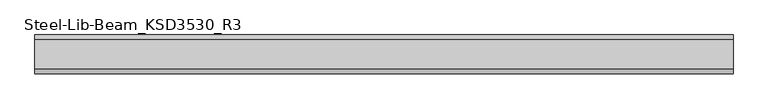
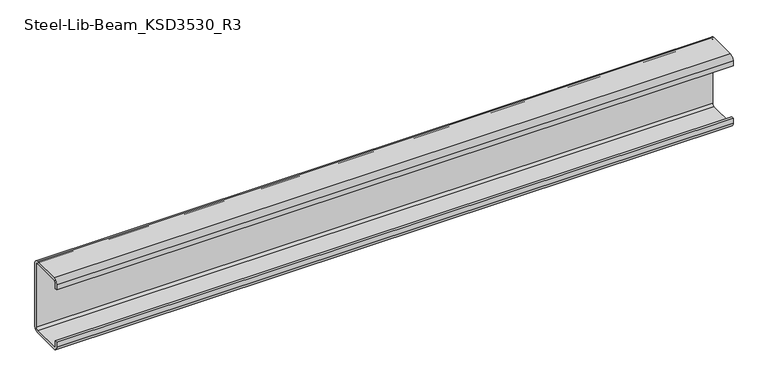
"""IFC4 building model written with IfcOpenShell, lengths in millimetres: beam geometry, Steel-Lib-Beam_KSD3530_R3 : BMS291_C-150×75x20x4.5."""

from ifc_helpers import new_model, si_unit, point, frame, frame_2d, origin, place, context, project, spatial, polyline, circle_curve, trimmed, segment, composite_curve, outline, extrude, source, transform, mapped, element, save


def steel_lib_beam_ksd3530_r3_1220318e(model_context):
    return source(origin(), model_context, "Body", "SweptSolid", [
        extrude(outline(composite_curve([segment(trimmed(circle_curve(frame_2d((-41.0, 66.0)), 9.0), [point((-50.0, 66.0))], [point((-41.0, 75.0))], False, "CARTESIAN"), True, "CONTINUOUS"), segment(polyline([(-41.0, 75.0), (16.0, 75.0)]), True, "CONTINUOUS"), segment(trimmed(circle_curve(frame_2d((16.0, 66.0)), 9.0), [point((16.0, 75.0))], [point((25.0, 66.0))], False, "CARTESIAN"), True, "CONTINUOUS"), segment(polyline([(25.0, 66.0), (25.0, -66.0)]), True, "CONTINUOUS"), segment(trimmed(circle_curve(frame_2d((16.0, -66.0)), 9.0), [point((25.0, -66.0))], [point((16.0, -75.0))], False, "CARTESIAN"), True, "CONTINUOUS"), segment(polyline([(16.0, -75.0), (-41.0, -75.0)]), True, "CONTINUOUS"), segment(trimmed(circle_curve(frame_2d((-41.0, -66.0)), 9.0), [point((-41.0, -75.0))], [point((-50.0, -66.0))], False, "CARTESIAN"), True, "CONTINUOUS"), segment(polyline([(-50.0, -66.0), (-50.0, -55.0), (-45.5, -55.0), (-45.5, -66.0)]), True, "CONTINUOUS"), segment(trimmed(circle_curve(frame_2d((-41.0, -66.0)), 4.5), [point((-45.5, -66.0))], [point((-41.0, -70.5))], True, "CARTESIAN"), True, "CONTINUOUS"), segment(polyline([(-41.0, -70.5), (16.0, -70.5)]), True, "CONTINUOUS"), segment(trimmed(circle_curve(frame_2d((16.0, -66.0)), 4.5), [point((16.0, -70.5))], [point((20.5, -66.0))], True, "CARTESIAN"), True, "CONTINUOUS"), segment(polyline([(20.5, -66.0), (20.5, 66.0)]), True, "CONTINUOUS"), segment(trimmed(circle_curve(frame_2d((16.0, 66.0)), 4.5), [point((20.5, 66.0))], [point((16.0, 70.5))], True, "CARTESIAN"), True, "CONTINUOUS"), segment(polyline([(16.0, 70.5), (-41.0, 70.5)]), True, "CONTINUOUS"), segment(trimmed(circle_curve(frame_2d((-41.0, 66.0)), 4.5), [point((-41.0, 70.5))], [point((-45.5, 66.0))], True, "CARTESIAN"), True, "CONTINUOUS"), segment(polyline([(-45.5, 66.0), (-45.5, 55.0), (-50.0, 55.0), (-50.0, 66.0)]), True, "CONTINUOUS")], self_intersect=False)), frame((-674.0, 0.0, 0.0), z_axis=(1.0, 0.0, 0.0), x_axis=(0.0, 1.0, 0.0)), (0.0, 0.0, 1.0), 1348.0),
    ])


if __name__ == "__main__":
    model = new_model("IFC4")
    model_context = context("Model", 3, world=origin())
    ifc_project = project(units=[si_unit("LENGTHUNIT", "METRE", prefix="MILLI")], contexts=[model_context])
    site = spatial("IfcSite", under=ifc_project)
    building = spatial("IfcBuilding", under=site)
    placement = place(None, origin())
    steel_lib_beam_ksd3530_r3_shape = steel_lib_beam_ksd3530_r3_1220318e(model_context)
    element("IfcBeam", 1, ObjectType="Steel-Lib-Beam_KSD3530_R3 : BMS291_C-150×75x20x4.5", at=placement, inside=building, context=model_context, shape_type="MappedRepresentation", body=[
        mapped(steel_lib_beam_ksd3530_r3_shape, transform((0.0, 0.0, 0.0), x_axis=(1.0, 0.0, 0.0), y_axis=(0.0, 1.0, 0.0), z_axis=(0.0, 0.0, 1.0))),
    ])
    save(model, "model.ifc")

# Revit data of these elements
# Type "Steel-Lib-Beam_KSD3530_R3 : BMS291_C-150×75x20x4.5"
#   Keynote = "C-150×75x20x4.5"
#   SteelWeight = "Light"
#   x = 0.0250 m
#   t1 = 0.0090 m
#   t = 0.0045 m
#   Surface Area = 0.629834 m²/m
#   Section Area = 13.9688 cm²
#   Mass per Unit Length = 10.9655 kg/m
#   C = 0.0200 m
#   A = 0.0750 m
#   Length [instance default] = 1.5000 m
#   H = 0.1500 m
#   hec_material4 [instance default] = none
#   hec_material3 [instance default] = none
#   hec_material2 [instance default] = none
#   hec_material1 [instance default] = none
#   Structural Material [instance default] = Metal - Steel - Light Gauge
#   Assembly Code = ""
# Element 1 (IfcBeam, "Steel-Lib-Beam_KSD3530_R3 : BMS291_C-150×75x20x4.5")
#   Structural Material = none
# Materials
#   "Metal - Steel - Light Gauge": class "Metal", colour RGB 247 247 247, transparency 0
